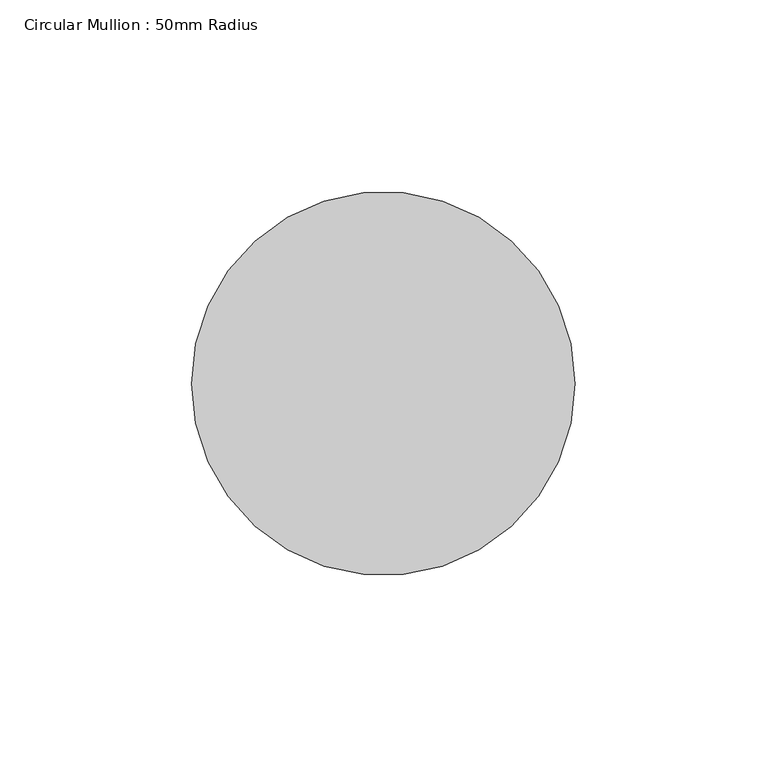
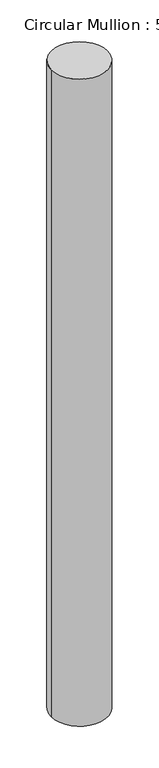
"""IFC4 building model written with IfcOpenShell, lengths in millimetres: member geometry, Circular Mullion : 50mm Radius."""

from ifc_helpers import new_model, si_unit, point, frame, origin, origin_2d, place, context, project, spatial, circle_curve, trimmed, segment, composite_curve, outline, extrude, source, transform, mapped, element, save


def circular_mullion_50mm_radius_61d3ef3d(model_context):
    return source(origin(), model_context, "Body", "SweptSolid", [
        extrude(outline(composite_curve([segment(trimmed(circle_curve(origin_2d(), 50.0), [point((50.0, 0.0))], [point((-50.0, 0.0))], False, "CARTESIAN"), True, "CONTINUOUS"), segment(trimmed(circle_curve(origin_2d(), 50.0), [point((-50.0, 0.0))], [point((50.0, 0.0))], False, "CARTESIAN"), True, "CONTINUOUS")], self_intersect=False)), frame((0.0, 0.0, -1211.3686593), z_axis=(0.0, 0.0, 1.0), x_axis=(1.0, 0.0, 0.0)), (0.0, 0.0, 1.0), 1211.3686593),
    ])


if __name__ == "__main__":
    model = new_model("IFC4")
    model_context = context("Model", 3, world=origin())
    ifc_project = project(units=[si_unit("LENGTHUNIT", "METRE", prefix="MILLI")], contexts=[model_context])
    site = spatial("IfcSite", under=ifc_project)
    building = spatial("IfcBuilding", under=site)
    placement = place(None, origin())
    circular_mullion_50mm_radius_shape = circular_mullion_50mm_radius_61d3ef3d(model_context)
    element("IfcMember", 1, ObjectType="Circular Mullion : 50mm Radius", at=placement, inside=building, context=model_context, shape_type="MappedRepresentation", body=[
        mapped(circular_mullion_50mm_radius_shape, transform((0.0, 0.0, 0.0), x_axis=(1.0, 0.0, 0.0), y_axis=(0.0, 1.0, 0.0), z_axis=(0.0, 0.0, 1.0))),
    ])
    save(model, "model.ifc")

# Revit data of these elements
# Type "Circular Mullion : 50mm Radius"
#   built-in parameter 1007350 = 0.164042 (stored number, unit not read)
# Element 1 (IfcMember, "Circular Mullion : 50mm Radius")
#   Materials on its faces: "Aluminium"
# Materials
#   "Aluminium": class "Metal", colour RGB 247 247 247, transparency 0, Description = "Aluminium 6061", Cost = 0
